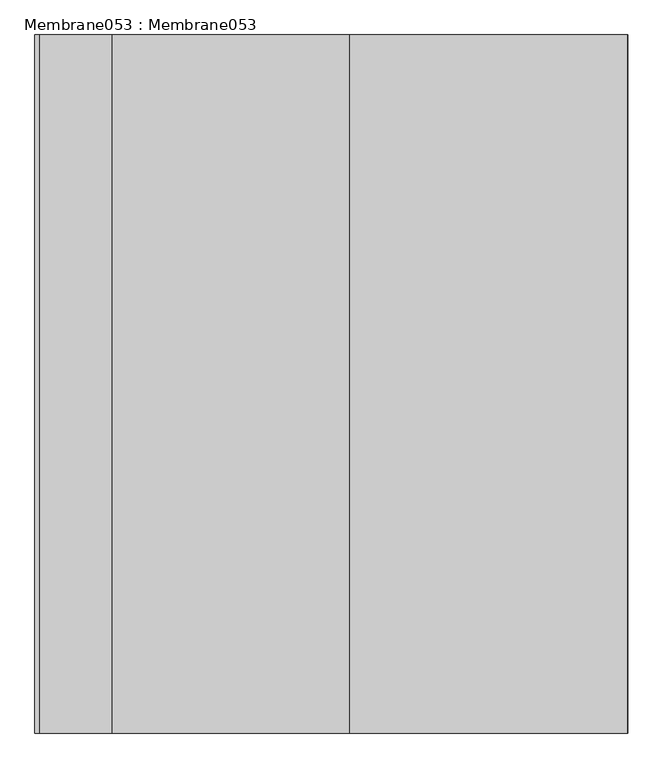
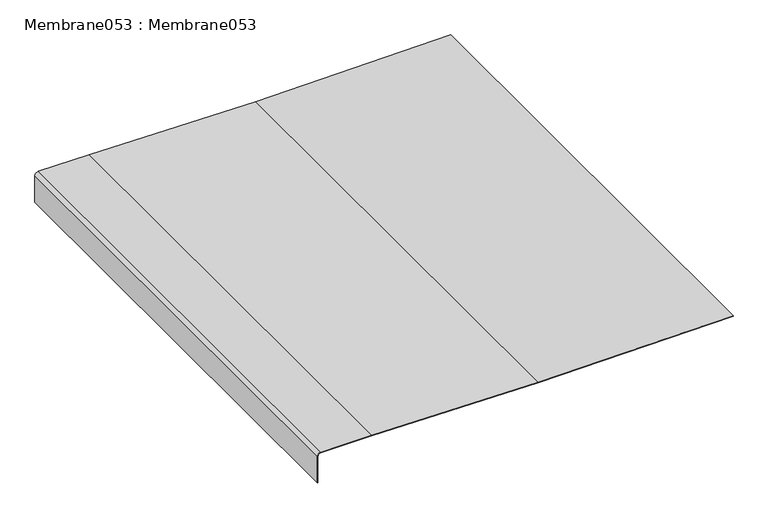
"""IFC4 building model written with IfcOpenShell, lengths in millimetres: proxy geometry, Membrane053 : Membrane053."""

from ifc_helpers import new_model, si_unit, point, frame, frame_2d, origin, place, context, project, spatial, polyline, circle_curve, trimmed, segment, composite_curve, outline, extrude, source, transform, mapped, element, save


def membrane053_membrane053_129f7b64(model_context):
    return source(origin(), model_context, "Body", "SweptSolid", [
        extrude(outline(composite_curve([segment(trimmed(circle_curve(frame_2d((40234.5370749, -2783.028052)), 12.0), [point((40234.5370749, -2795.028052))], [point((40246.5370749, -2783.028052))], True, "CARTESIAN"), True, "CONTINUOUS"), segment(polyline([(40246.5370749, -2783.028052), (40246.5370749, -2575.7595485), (40236.7392216, -1894.9487955), (40246.5370749, -1098.4673881), (40248.5369236, -1098.4919891), (40238.7393987, -1894.9467057), (40248.5370749, -2575.7451577), (40248.5370749, -2783.028052)]), True, "CONTINUOUS"), segment(trimmed(circle_curve(frame_2d((40234.5370749, -2783.028052)), 14.0), [point((40248.5370749, -2783.028052))], [point((40234.5370749, -2797.028052))], False, "CARTESIAN"), True, "CONTINUOUS"), segment(polyline([(40234.5370749, -2797.028052), (40120.9129128, -2797.028052), (40120.9129128, -2795.028052), (40234.5370749, -2795.028052)]), True, "CONTINUOUS")], self_intersect=False)), frame((0.0, -1052.8906574, 0.0), z_axis=(0.0, 1.0, 0.0), x_axis=(0.0, 0.0, 1.0)), (0.0, 0.0, 1.0), 2000.0),
    ])


if __name__ == "__main__":
    model = new_model("IFC4")
    model_context = context("Model", 3, world=origin())
    ifc_project = project(units=[si_unit("LENGTHUNIT", "METRE", prefix="MILLI")], contexts=[model_context])
    site = spatial("IfcSite", under=ifc_project)
    building = spatial("IfcBuilding", under=site)
    placement = place(None, origin())
    membrane053_membrane053_shape = membrane053_membrane053_129f7b64(model_context)
    element("IfcBuildingElementProxy", 1, Name="Membrane053 : Membrane053", ObjectType="Membrane053 : Membrane053", at=placement, inside=building, context=model_context, shape_type="MappedRepresentation", body=[
        mapped(membrane053_membrane053_shape, transform((0.0, 0.0, 0.0), x_axis=(1.0, 0.0, 0.0), y_axis=(0.0, 1.0, 0.0), z_axis=(0.0, 0.0, 1.0))),
    ])
    save(model, "model.ifc")

# Revit data of these elements
# Type "Membrane053 : Membrane053"
#   NameOverride = "Membrane053"
# Element 1 (IfcBuildingElementProxy, "Membrane053 : Membrane053")
#   Materials on its faces: "THREE PLY BUILT UP ROOF MEMBRANE"
# Materials
#   "THREE PLY BUILT UP ROOF MEMBRANE": class "Unassigned", colour RGB 63 63 63, transparency 0
